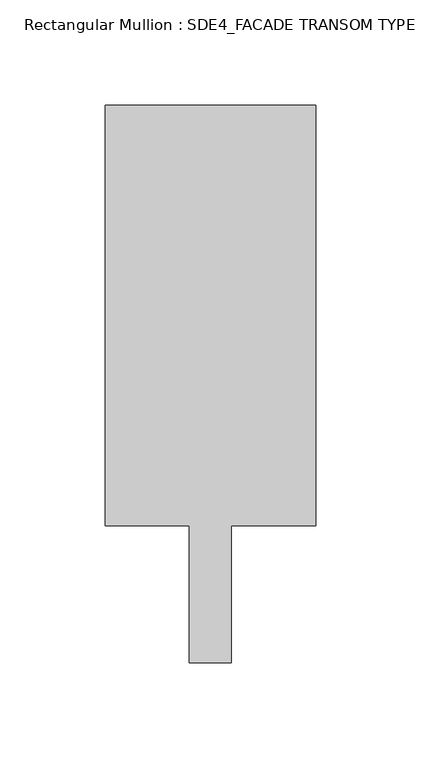
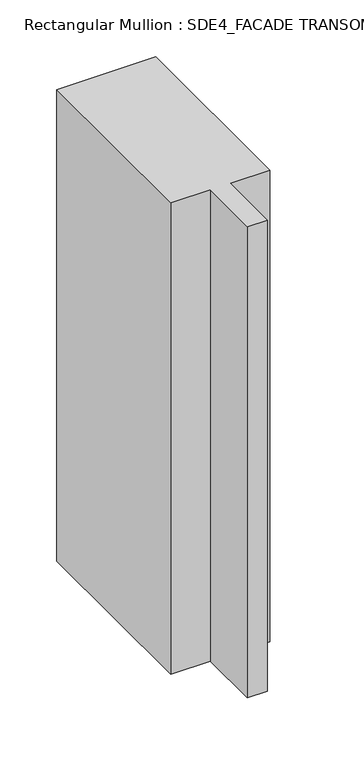
"""IFC4 building model written with IfcOpenShell, lengths in millimetres: member geometry, Rectangular Mullion : SDE4_FACADE TRANSOM TYPE 2."""

from ifc_helpers import new_model, si_unit, frame, origin, place, context, project, spatial, polyline, outline, extrude, source, transform, mapped, element, save


def rectangular_mullion_sde4_facade_transom_type_2_eb508603(model_context):
    return source(origin(), model_context, "Body", "SweptSolid", [
        extrude(outline(polyline([(50.0, 132.5), (50.0, -67.5), (10.0, -67.5), (10.0, -132.5), (-10.0, -132.5), (-10.0, -67.5), (-50.0, -67.5), (-50.0, 132.5), (50.0, 132.5)])), frame((0.0, 0.0, -505.06364), z_axis=(0.0, 0.0, 1.0), x_axis=(1.0, 0.0, 0.0)), (0.0, 0.0, 1.0), 505.06364),
    ])


if __name__ == "__main__":
    model = new_model("IFC4")
    model_context = context("Model", 3, world=origin())
    ifc_project = project(units=[si_unit("LENGTHUNIT", "METRE", prefix="MILLI")], contexts=[model_context])
    site = spatial("IfcSite", under=ifc_project)
    building = spatial("IfcBuilding", under=site)
    placement = place(None, origin())
    rectangular_mullion_sde4_facade_transom_type_2_shape = rectangular_mullion_sde4_facade_transom_type_2_eb508603(model_context)
    element("IfcMember", 1, ObjectType="Rectangular Mullion : SDE4_FACADE TRANSOM TYPE 2", at=placement, inside=building, context=model_context, shape_type="MappedRepresentation", body=[
        mapped(rectangular_mullion_sde4_facade_transom_type_2_shape, transform((0.0, 0.0, 0.0), x_axis=(1.0, 0.0, 0.0), y_axis=(0.0, 1.0, 0.0), z_axis=(0.0, 0.0, 1.0))),
    ])
    save(model, "model.ifc")

# Revit data of these elements
# Type "Rectangular Mullion : SDE4_FACADE TRANSOM TYPE 2"
#   built-in parameter 1007322 = 0.869423 (stored number, unit not read)
#   built-in parameter 1007321 = 0.164042 (stored number, unit not read)
#   built-in parameter 1007320 = 0.164042 (stored number, unit not read)
